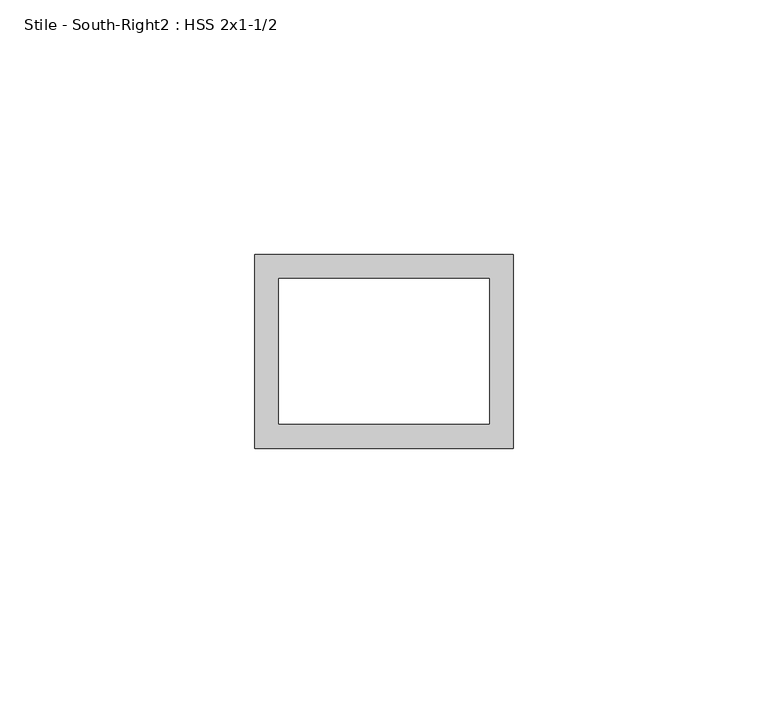
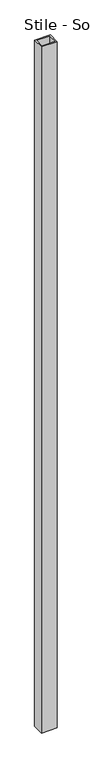
"""IFC4 building model written with IfcOpenShell, lengths in millimetres: proxy geometry, Stile - South-Right2 : HSS 2x1-1/2."""

from ifc_helpers import new_model, si_unit, frame, origin, place, context, project, spatial, polyline, outline, extrude, source, transform, mapped, element, save


def stile_south_right2_hss_2x1_1_2_5f68abb1(model_context):
    return source(origin(), model_context, "Body", "SweptSolid", [
        extrude(outline(polyline([(587365.8934739, -533937.9163841), (587416.6934739, -533937.9163841), (587416.6934739, -533976.0163841), (587365.8934739, -533976.0163841), (587365.8934739, -533937.9163841)]), holes=[polyline([(587370.6559739, -533942.6788841), (587370.6559739, -533971.2538841), (587411.9309739, -533971.2538841), (587411.9309739, -533942.6788841), (587370.6559739, -533942.6788841)])]), frame((0.0, 0.0, 50.8), z_axis=(0.0, 0.0, 1.0), x_axis=(1.0, 0.0, 0.0)), (0.0, 0.0, 1.0), 2349.5),
    ])


if __name__ == "__main__":
    model = new_model("IFC4")
    model_context = context("Model", 3, world=origin())
    ifc_project = project(units=[si_unit("LENGTHUNIT", "METRE", prefix="MILLI")], contexts=[model_context])
    site = spatial("IfcSite", under=ifc_project)
    building = spatial("IfcBuilding", under=site)
    placement = place(None, origin())
    stile_south_right2_hss_2x1_1_2_shape = stile_south_right2_hss_2x1_1_2_5f68abb1(model_context)
    element("IfcBuildingElementProxy", 1, Name="Stile - South-Right2 : HSS 2x1-1/2", ObjectType="Stile - South-Right2 : HSS 2x1-1/2", at=placement, inside=building, context=model_context, shape_type="MappedRepresentation", body=[
        mapped(stile_south_right2_hss_2x1_1_2_shape, transform((0.0, 0.0, 0.0), x_axis=(1.0, 0.0, 0.0), y_axis=(0.0, 1.0, 0.0), z_axis=(0.0, 0.0, 1.0))),
    ])
    save(model, "model.ifc")

# Revit data of these elements
# Element 1 (IfcBuildingElementProxy, "Stile - South-Right2 : HSS 2x1-1/2")
#   Materials on its faces: "1-1/2\"X2\" GALV. STL HSS TUBING"
# Materials
#   "1-1/2\"X2\" GALV. STL HSS TUBING": class "Generic", colour RGB 211 211 207, transparency 0, Cost = 0
